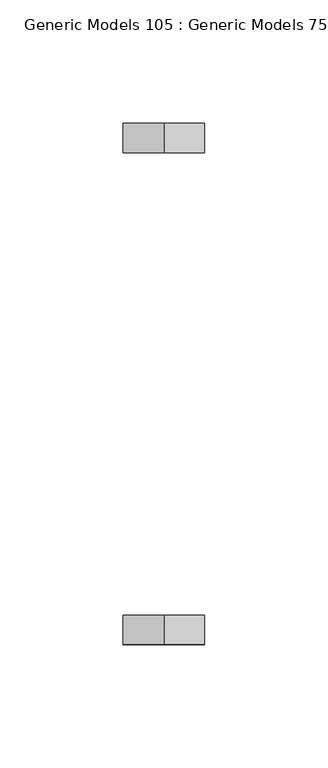
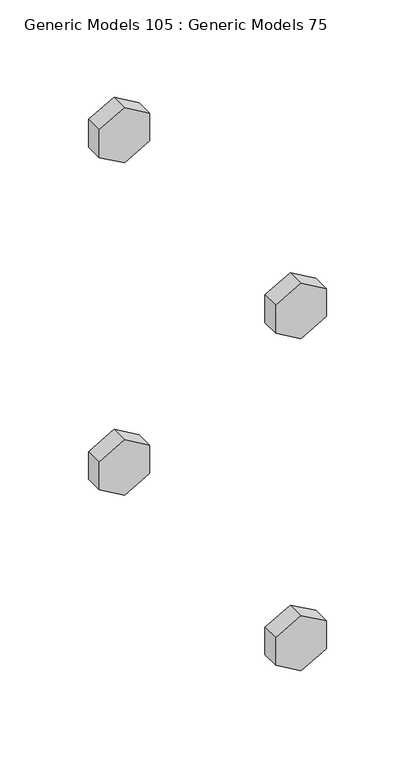
"""IFC4 building model written with IfcOpenShell, lengths in millimetres: proxy geometry, Generic Models 105 : Generic Models 75."""

from ifc_helpers import new_model, si_unit, frame, origin, place, context, project, spatial, polyline, outline, extrude, source, transform, mapped, element, save


def generic_models_105_generic_models_75_ef56f7d8(model_context):
    return source(origin(), model_context, "Body", "SweptSolid", [
        extrude(outline(polyline([(268824.075, 31991.9073871), (268843.125, 31991.9073871), (268852.65, 31975.4096032), (268843.125, 31958.9118192), (268824.075, 31958.9118192), (268814.55, 31975.4096032), (268824.075, 31991.9073871)])), frame((0.0, 30668.7719112, 0.0), z_axis=(0.0, 1.0, 0.0), x_axis=(0.0, 0.0, 1.0)), (0.0, 0.0, 1.0), 11.90625),
        extrude(outline(polyline([(269052.675, 31991.9073871), (269071.725, 31991.9073871), (269081.25, 31975.4096032), (269071.725, 31958.9118192), (269052.675, 31958.9118192), (269043.15, 31975.4096032), (269052.675, 31991.9073871)])), frame((0.0, 30668.7719112, 0.0), z_axis=(0.0, 1.0, 0.0), x_axis=(0.0, 0.0, 1.0)), (0.0, 0.0, 1.0), 11.90625),
        extrude(outline(polyline([(268824.075, 31991.9073871), (268843.125, 31991.9073871), (268852.65, 31975.4096032), (268843.125, 31958.9118192), (268824.075, 31958.9118192), (268814.55, 31975.4096032), (268824.075, 31991.9073871)])), frame((0.0, 30868.0031612, 0.0), z_axis=(0.0, 1.0, 0.0), x_axis=(0.0, 0.0, 1.0)), (0.0, 0.0, 1.0), 11.90625),
        extrude(outline(polyline([(269052.675, 31991.9073871), (269071.725, 31991.9073871), (269081.25, 31975.4096032), (269071.725, 31958.9118192), (269052.675, 31958.9118192), (269043.15, 31975.4096032), (269052.675, 31991.9073871)])), frame((0.0, 30868.0031612, 0.0), z_axis=(0.0, 1.0, 0.0), x_axis=(0.0, 0.0, 1.0)), (0.0, 0.0, 1.0), 11.90625),
    ])


if __name__ == "__main__":
    model = new_model("IFC4")
    model_context = context("Model", 3, world=origin())
    ifc_project = project(units=[si_unit("LENGTHUNIT", "METRE", prefix="MILLI")], contexts=[model_context])
    site = spatial("IfcSite", under=ifc_project)
    building = spatial("IfcBuilding", under=site)
    placement = place(None, origin())
    generic_models_105_generic_models_75_shape = generic_models_105_generic_models_75_ef56f7d8(model_context)
    element("IfcBuildingElementProxy", 1, Name="Generic Models 105 : Generic Models 75", ObjectType="Generic Models 105 : Generic Models 75", at=placement, inside=building, context=model_context, shape_type="MappedRepresentation", body=[
        mapped(generic_models_105_generic_models_75_shape, transform((0.0, 0.0, 0.0), x_axis=(1.0, 0.0, 0.0), y_axis=(0.0, 1.0, 0.0), z_axis=(0.0, 0.0, 1.0))),
    ])
    save(model, "model.ifc")
